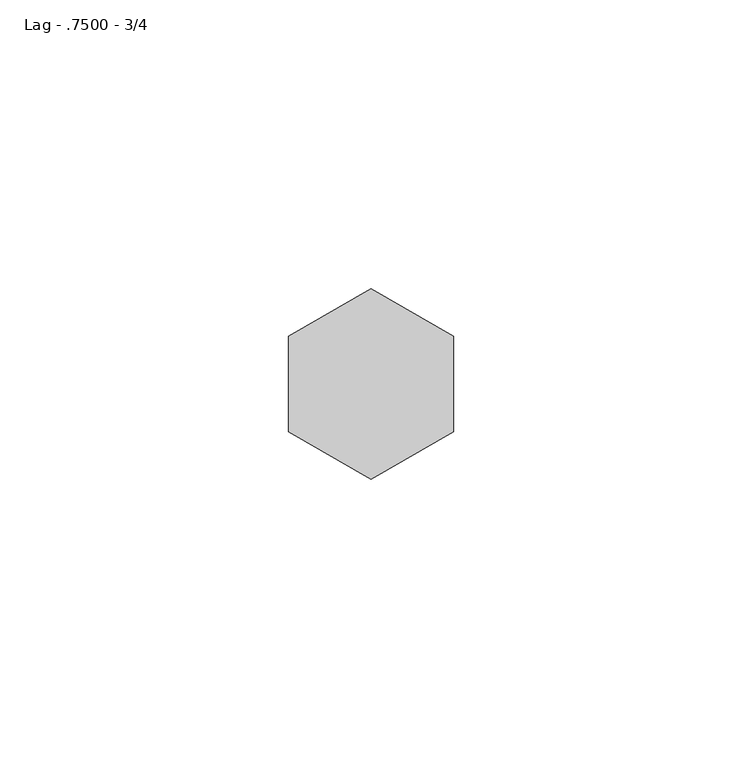
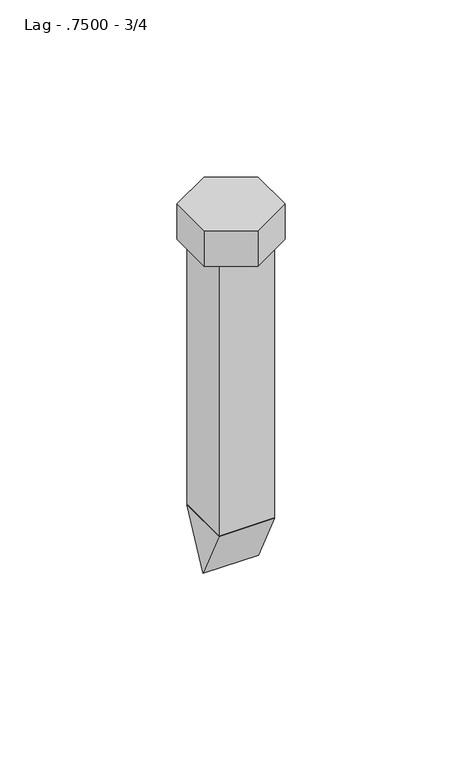
"""IFC4 building model written with IfcOpenShell, lengths in millimetres: fastener geometry, 060523 - W_P_C - Fastenings - Generic - SQUARE : Lag - .7500 - 3/4."""

from ifc_helpers import new_model, si_unit, frame, origin, origin_with_axes, place, context, project, spatial, polyline, outline, extrude, source, transform, mapped, element, save


def lag_7500_3_4_9180f7ef(model_context):
    return source(origin(), model_context, "Body", "SweptSolid", [
        extrude(outline(polyline([(0.0, -121.1460937), (-9.7730469, -101.6), (9.7730469, -101.6), (0.0, -121.1460937)])), frame((-9.7730469, 0.0, 0.0), z_axis=(1.0, 0.0, 0.0), x_axis=(0.0, 1.0, 0.0)), (0.0, 0.0, 1.0), 19.5460938),
        extrude(outline(polyline([(-14.2875, 8.248892), (0.0, 16.4977839), (14.2875, 8.248892), (14.2875, -8.248892), (0.0, -16.4977839), (-14.2875, -8.248892), (-14.2875, 8.248892)])), origin_with_axes(), (0.0, 0.0, 1.0), 13.2953125),
        extrude(outline(polyline([(-9.7730469, 9.7730469), (9.7730469, 9.7730469), (9.7730469, -9.7730469), (-9.7730469, -9.7730469), (-9.7730469, 9.7730469)])), frame((0.0, 0.0, -101.6), z_axis=(0.0, 0.0, 1.0), x_axis=(1.0, 0.0, 0.0)), (0.0, 0.0, 1.0), 101.6),
    ])


if __name__ == "__main__":
    model = new_model("IFC4")
    model_context = context("Model", 3, world=origin())
    ifc_project = project(units=[si_unit("LENGTHUNIT", "METRE", prefix="MILLI")], contexts=[model_context])
    site = spatial("IfcSite", under=ifc_project)
    building = spatial("IfcBuilding", under=site)
    placement = place(None, origin())
    lag_7500_3_4_shape = lag_7500_3_4_9180f7ef(model_context)
    element("IfcFastener", 1, ObjectType="060523 - W_P_C - Fastenings - Generic - SQUARE : Lag - .7500 - 3/4", at=placement, inside=building, context=model_context, shape_type="MappedRepresentation", body=[
        mapped(lag_7500_3_4_shape, transform((0.0, 0.0, 0.0), x_axis=(1.0, 0.0, 0.0), y_axis=(0.0, 1.0, 0.0), z_axis=(0.0, 0.0, 1.0))),
    ])
    save(model, "model.ifc")

# Revit data of these elements
# Type "060523 - W_P_C - Fastenings - Generic - SQUARE : Lag - .7500 - 3/4"
#   Washer_Thickness = 0' - 0.17448"
#   Washer Radius = 0' - 0.9082"
#   Washer Offset - Head = 0' - 0"
#   Washer Offset = 0' - 0"
#   Thickness_of_Substrate [instance default] = 0' - 1"
#   Side = 0' - 0.65039"
#   Radius = 0' - 0.38477"
#   Length [instance default] = 0' - 4"
#   Head Size = 0' - 1 1/8"
#   Head Radius = 0' - 0 9/16"
#   Head Height = 0' - 0 67/128"
#   Double Diameter = 0' - 1 69/128"
#   Diameter = 0' - 0 197/256"
#   Default Elevation = 4' - 0"
#   Washer_Nut_Visibility = no
#   Washer_Head_Visibility = no
#   Round_Head_Visibility = no
#   Point Visibility = yes
#   Nut_Visibility = no
#   Hex_Head_Visiblilty = yes
#   Washer Material = none
#   Bolt Material (Size) = AT SILL - FASTENER AT 24" O.C.
# Element 1 (IfcFastener, "060523 - W_P_C - Fastenings - Generic - SQUARE : Lag - .7500 - 3/4")
#   Materials on its faces: "AT SILL - FASTENER AT 24\" O.C."
# Materials
#   "AT SILL - FASTENER AT 24\" O.C.": class "Generic", colour RGB 120 120 120, transparency 0, Cost = 0
